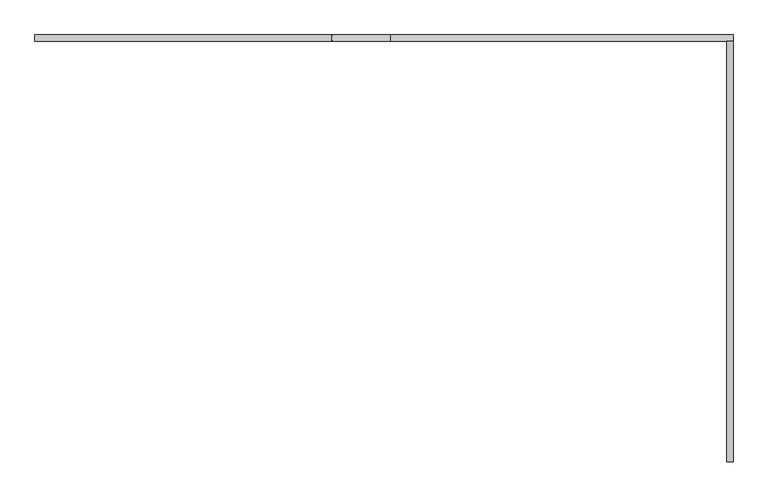
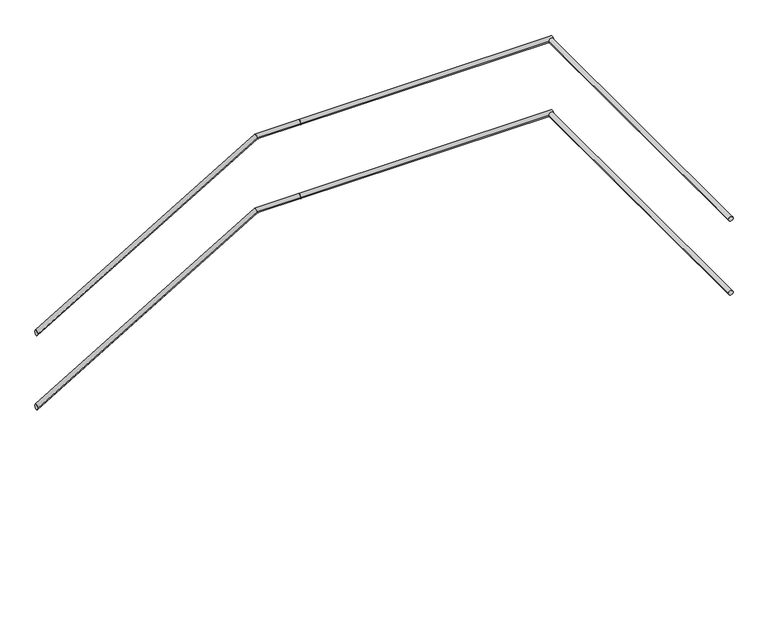
"""IFC4 building model written with IfcOpenShell, lengths in millimetres: railing geometry."""

import ifcopenshell
import ifcopenshell.guid

model = None  # the IFC model being written
_history = None  # IfcOwnerHistory: only IFC2X3 demands one
_inside = {}  # id of a spatial element -> (the spatial element, [elements in it])
_under = {}  # id of a project, library or spatial element -> (it, [spatial elements below it])
_declared = {}  # id of a project -> (the project, [libraries it declares])
_typed = {}  # id of a type object -> (the type object, [elements of that type])
_made_of = {}  # id of a material, layer set ... -> (it, [elements and type objects made of it])


def new_model(schema):
    """Start an empty IFC model of exactly this schema.

    Asked for "IFC4X3", IfcOpenShell would pick the latest addendum, in which some entities
    have other attributes; the version numbers below select the first issue.
    IFC2X3 requires an IfcOwnerHistory on every rooted entity: one is made here for all.
    """
    global model, _history
    if schema == "IFC4X3":
        model = ifcopenshell.file(schema_version=(4, 3, 0, 0))
    else:
        model = ifcopenshell.file(schema=schema)
    _inside.clear()
    _under.clear()
    _declared.clear()
    _typed.clear()
    _made_of.clear()
    _history = None
    if model.schema == "IFC2X3":
        org = make("IfcOrganization", Name="unknown")
        user = make(
            "IfcPersonAndOrganization",
            ThePerson=make("IfcPerson", FamilyName="unknown"),
            TheOrganization=org,
        )
        app = make(
            "IfcApplication",
            ApplicationDeveloper=org,
            Version="unknown",
            ApplicationFullName="unknown",
            ApplicationIdentifier="unknown",
        )
        _history = make(
            "IfcOwnerHistory",
            OwningUser=user,
            OwningApplication=app,
            ChangeAction="ADDED",
            CreationDate=0,
        )
    return model


def make(cls, **values):
    """One entity of the class cls with the attributes given. An attribute that is None is left unset."""
    return model.create_entity(
        cls, **{name: value for name, value in values.items() if value is not None}
    )


def rooted(cls, **values):
    """An entity with a GlobalId (a new one), such as an element, a storey or a relation."""
    return make(cls, GlobalId=ifcopenshell.guid.new(), OwnerHistory=_history, **values)


def si_unit(unit_type, name, prefix=None):
    """IfcSIUnit, for example si_unit("LENGTHUNIT", "METRE", prefix="MILLI")."""
    return make("IfcSIUnit", UnitType=unit_type, Prefix=prefix, Name=name)


def assignment(units):
    """IfcUnitAssignment: the units of a project."""
    return None if units is None else make("IfcUnitAssignment", Units=units)


def point(xyz):
    """IfcCartesianPoint."""
    return None if xyz is None else make("IfcCartesianPoint", Coordinates=xyz)


def direction(xyz):
    """IfcDirection."""
    return None if xyz is None else make("IfcDirection", DirectionRatios=xyz)


def frame(location, z_axis=None, x_axis=None):
    """IfcAxis2Placement3D, a coordinate frame: its origin and axes. An axis left out is left unset."""
    return make(
        "IfcAxis2Placement3D",
        Location=point(location),
        Axis=direction(z_axis),
        RefDirection=direction(x_axis),
    )


def origin():
    """The frame at (0, 0, 0) with its axes left unset."""
    return frame((0.0, 0.0, 0.0))


def place(relative_to, where):
    """IfcLocalPlacement: puts the frame where relative to a parent placement (None: the world)."""
    return make(
        "IfcLocalPlacement", PlacementRelTo=relative_to, RelativePlacement=where
    )


def context(
    kind, dimensions, precision=None, world=None, true_north=None, identifier=None
):
    """IfcGeometricRepresentationContext, for example the 3D "Model" context."""
    return make(
        "IfcGeometricRepresentationContext",
        ContextIdentifier=identifier,
        ContextType=kind,
        CoordinateSpaceDimension=dimensions,
        Precision=precision,
        WorldCoordinateSystem=world,
        TrueNorth=true_north,
    )


def project(units=None, contexts=None):
    """IfcProject with its units and contexts."""
    return rooted(
        "IfcProject",
        Name="project",
        RepresentationContexts=contexts,
        UnitsInContext=assignment(units),
    )


def spatial(cls, under=None, at=None, **own):
    """A site, building, storey or space (cls), placed at a placement, below another one or the project."""
    s = rooted(cls, ObjectPlacement=at, **own)
    if under is not None:
        _under.setdefault(under.id(), (under, []))[1].append(s)
    return s


def circle_curve(where, radius):
    """IfcCircle in the frame where."""
    return make("IfcCircle", Position=where, Radius=radius)


def ellipse_curve(where, semi_axis1, semi_axis2):
    """IfcEllipse in the frame where."""
    return make(
        "IfcEllipse", Position=where, SemiAxis1=semi_axis1, SemiAxis2=semi_axis2
    )


def shape(context_of_items, identifier, shape_type, items):
    """IfcShapeRepresentation: the items that make up one representation, for example the "Body"."""
    return make(
        "IfcShapeRepresentation",
        ContextOfItems=context_of_items,
        RepresentationIdentifier=identifier,
        RepresentationType=shape_type,
        Items=items,
    )


def source(mapping_origin, context_of_items, identifier, shape_type, items):
    """IfcRepresentationMap: a shape defined once, which mapped items show again and again."""
    return make(
        "IfcRepresentationMap",
        MappingOrigin=mapping_origin,
        MappedRepresentation=shape(context_of_items, identifier, shape_type, items),
    )


def transform(
    local_origin,
    x_axis=None,
    y_axis=None,
    z_axis=None,
    scale=None,
    scale2=None,
    scale3=None,
    uniform=True,
):
    """IfcCartesianTransformationOperator3D, or its non-uniform kind. x_axis, y_axis, z_axis: its Axis1, 2, 3."""
    if uniform:
        return make(
            "IfcCartesianTransformationOperator3D",
            Axis1=direction(x_axis),
            Axis2=direction(y_axis),
            LocalOrigin=point(local_origin),
            Scale=scale,
            Axis3=direction(z_axis),
        )
    return make(
        "IfcCartesianTransformationOperator3DnonUniform",
        Axis1=direction(x_axis),
        Axis2=direction(y_axis),
        LocalOrigin=point(local_origin),
        Scale=scale,
        Axis3=direction(z_axis),
        Scale2=scale2,
        Scale3=scale3,
    )


def mapped(mapping_source, mapping_target):
    """IfcMappedItem: shows the shape of a source again, moved by a transform."""
    return make(
        "IfcMappedItem", MappingSource=mapping_source, MappingTarget=mapping_target
    )


def made_of(thing, what):
    """Note that an element or type object is made of a material, layer set ...; save() writes the relation."""
    if what is not None:
        _made_of.setdefault(what.id(), (what, []))[1].append(thing)
    return thing


def element(
    cls,
    number,
    at=None,
    inside=None,
    cuts=None,
    type_object=None,
    material=None,
    context=None,
    identifier="Body",
    shape_type=None,
    held_by="IfcProductDefinitionShape",
    body=None,
    shapes=None,
    **own,
):
    """One element of the class cls, such as IfcWall. Its Tag is "e" and its number.

    at: its placement. inside: the storey or other place that contains it. cuts: it is an
    opening in that element (IfcRelVoidsElement). A single representation is given by context,
    identifier, shape_type and body (its items); several are given by shapes. held_by: the class
    of the entity that holds the representations. save() writes the other relations.
    """
    e = rooted(cls, Tag="e%d" % number, ObjectPlacement=at, **own)
    if body is not None:
        shapes = [shape(context, identifier, shape_type, body)]
    if shapes is not None:
        e.Representation = make(held_by, Representations=shapes)
    if inside is not None:
        _inside.setdefault(inside.id(), (inside, []))[1].append(e)
    if cuts is not None:
        rooted(
            "IfcRelVoidsElement", RelatingBuildingElement=cuts, RelatedOpeningElement=e
        )
    if type_object is not None:
        _typed.setdefault(type_object.id(), (type_object, []))[1].append(e)
    return made_of(e, material)


def aggregate(whole, parts):
    """IfcRelAggregates: a whole, such as a stair, and the parts it consists of."""
    return rooted("IfcRelAggregates", RelatingObject=whole, RelatedObjects=parts)


def save(model, path):
    """Write the relations noted so far, then the file.

    IfcRelAggregates (storeys below a building ...), IfcRelContainedInSpatialStructure (elements
    in a storey), IfcRelDefinesByType, IfcRelAssociatesMaterial and IfcRelDeclares: one each for
    every whole, place, type object, material and project.
    """
    for whole, parts in _under.values():
        aggregate(whole, parts)
    for where, things in _inside.values():
        rooted(
            "IfcRelContainedInSpatialStructure",
            RelatedElements=things,
            RelatingStructure=where,
        )
    for kind, things in _typed.values():
        rooted("IfcRelDefinesByType", RelatedObjects=things, RelatingType=kind)
    for what, things in _made_of.values():
        rooted("IfcRelAssociatesMaterial", RelatedObjects=things, RelatingMaterial=what)
    for by, libraries in _declared.values():
        rooted("IfcRelDeclares", RelatingContext=by, RelatedDefinitions=libraries)
    model.write(path)


def plane_surface(at):
    """IfcPlane: the flat surface through the origin of the frame at, square to its z axis."""
    return make("IfcPlane", Position=at)


def cylinder_surface(at, radius):
    """IfcCylindricalSurface: all points at the distance radius from the z axis of the frame at."""
    return make("IfcCylindricalSurface", Position=at, Radius=radius)


def advanced_brep(points, edges, surfaces, faces):
    """IfcAdvancedBrep: a solid bounded by faces that lie on surfaces and meet in shared edges.

    An edge is (start, end): straight between two places in points (the first is 0);
    or (start, end, curve); or (start, end, curve, False) where it runs against its curve.
    A face is (place in surfaces, loops), or (place, loops, False) where it looks against
    its surface's normal. A loop lists edges by number (the first is 1), with a minus sign
    where the edge is run from its end to its start. The first loop is the outer one.
    """
    corners = [point(p) for p in points]
    vertices = [make("IfcVertexPoint", VertexGeometry=c) for c in corners]
    made = []
    for start, end, *more in edges:
        made.append(
            make(
                "IfcEdgeCurve",
                EdgeStart=vertices[start],
                EdgeEnd=vertices[end],
                EdgeGeometry=more[0] if more else make("IfcPolyline", Points=[corners[start], corners[end]]),
                SameSense=more[1] if len(more) > 1 else True,
            )
        )
    hull = []
    for where, loops, *sense in faces:
        bounds = []
        for j, loop in enumerate(loops):
            ring = [make("IfcOrientedEdge", EdgeElement=made[abs(k) - 1], Orientation=k > 0) for k in loop]
            bounds.append(
                make(
                    "IfcFaceOuterBound" if j == 0 else "IfcFaceBound",
                    Bound=make("IfcEdgeLoop", EdgeList=ring),
                    Orientation=True,
                )
            )
        hull.append(make("IfcAdvancedFace", Bounds=bounds, FaceSurface=surfaces[where], SameSense=sense[0] if sense else True))
    return make("IfcAdvancedBrep", Outer=make("IfcClosedShell", CfsFaces=hull))


def railing_b1a865fd(model_context):
    return source(origin(), model_context, "Body", "AdvancedBrep", [
        advanced_brep(
        [(45466.7161135, 23749.5208589, 1734.9618634), (45496.7161135, 23749.5208589, 1734.9618634), (45466.7161135, 25734.1208589, 1734.9618634), (45496.7161135, 25734.1208589, 1734.9618634)],
        [
            (0, 1, circle_curve(frame((45481.7161135, 23749.5208589, 1734.9618634), z_axis=(0.0, -1.0, 0.0), x_axis=(1.0, 0.0, 0.0)), 15.0)),
            (1, 0, circle_curve(frame((45481.7161135, 23749.5208589, 1734.9618634), z_axis=(0.0, -1.0, 0.0), x_axis=(1.0, 0.0, 0.0)), 15.0)),
            (2, 3, circle_curve(frame((45481.7161135, 25734.1208589, 1734.9618634), z_axis=(0.0, 1.0, 0.0), x_axis=(1.0, 0.0, 0.0)), 15.0)),
            (3, 2, circle_curve(frame((45481.7161135, 25734.1208589, 1734.9618634), z_axis=(0.0, 1.0, 0.0), x_axis=(1.0, 0.0, 0.0)), 15.0)),
            (0, 2),
            (3, 1),
        ],
        [
            plane_surface(frame((45481.7161135, 23749.5208589, 1749.9618634), z_axis=(0.0, -1.0, 0.0), x_axis=(0.0, 0.0, 1.0))),
            plane_surface(frame((45481.7161135, 25734.1208589, 1749.9618634), z_axis=(0.0, 1.0, 0.0), x_axis=(0.0, 0.0, 1.0))),
            cylinder_surface(frame((45481.7161135, 23749.5208589, 1734.9618634), z_axis=(0.0, -1.0, 0.0), x_axis=(1.0, 0.0, 0.0)), 15.0),
        ],
        [
            (0, [[1, 2]]),
            (1, [[3, 4]]),
            (2, [[-1, 5, -4, 6]]),
            (2, [[-2, -6, -3, -5]]),
        ],
    ),
        advanced_brep(
        [(45496.7161135, 25734.1208589, 1734.9618634), (45496.7161135, 25764.1208589, 1734.9618634), (43882.1161135, 25734.1208589, 1734.9618634), (43882.1161135, 25764.1208589, 1734.9618634)],
        [
            (0, 1, circle_curve(frame((45496.7161135, 25749.1208589, 1734.9618634), z_axis=(1.0, 0.0, 0.0), x_axis=(0.0, 1.0, 0.0)), 15.0)),
            (1, 0, circle_curve(frame((45496.7161135, 25749.1208589, 1734.9618634), z_axis=(1.0, 0.0, 0.0), x_axis=(0.0, 1.0, 0.0)), 15.0)),
            (2, 3, circle_curve(frame((43882.1161135, 25749.1208589, 1734.9618634), z_axis=(-1.0, 0.0, 0.0), x_axis=(0.0, 1.0, 0.0)), 15.0)),
            (3, 2, circle_curve(frame((43882.1161135, 25749.1208589, 1734.9618634), z_axis=(-1.0, 0.0, 0.0), x_axis=(0.0, 1.0, 0.0)), 15.0)),
            (0, 2),
            (3, 1),
        ],
        [
            plane_surface(frame((45496.7161135, 25749.1208589, 1749.9618634), z_axis=(1.0, 0.0, 0.0), x_axis=(0.0, -1.0, 0.0))),
            plane_surface(frame((43882.1161135, 25749.1208589, 1749.9618634), z_axis=(-1.0, 0.0, 0.0), x_axis=(0.0, -1.0, 0.0))),
            cylinder_surface(frame((45496.7161135, 25749.1208589, 1734.9618634), z_axis=(1.0, 0.0, 0.0), x_axis=(0.0, 1.0, 0.0)), 15.0),
        ],
        [
            (0, [[1, 2]]),
            (1, [[3, 4]]),
            (2, [[-1, 5, -4, 6]]),
            (2, [[-2, -6, -3, -5]]),
        ],
    ),
        advanced_brep(
        [(43882.1161135, 25734.1208589, 1734.9618634), (43882.1161135, 25764.1208589, 1734.9618634), (43606.242552, 25734.1208589, 1734.9618634), (43606.242552, 25764.1208589, 1734.9618634), (42202.1161135, 25734.1208589, 899.1723166), (42202.1161135, 25764.1208589, 899.1723166)],
        [
            (0, 1, circle_curve(frame((43882.1161135, 25749.1208589, 1734.9618634), z_axis=(1.0, 0.0, 0.0), x_axis=(0.0, 1.0, 0.0)), 15.0)),
            (1, 0, circle_curve(frame((43882.1161135, 25749.1208589, 1734.9618634), z_axis=(1.0, 0.0, 0.0), x_axis=(0.0, 1.0, 0.0)), 15.0)),
            (0, 2),
            (2, 3, ellipse_curve(frame((43606.242552, 25749.1208589, 1734.9618634), z_axis=(0.9641817474962143, 0.0, 0.2652424509673111), x_axis=(0.265242450967311, 0.0, -0.9641817474962144)), 15.5572329, 15.0)),
            (3, 1),
            (3, 2, ellipse_curve(frame((43606.242552, 25749.1208589, 1734.9618634), z_axis=(0.9641817474962143, 0.0, 0.2652424509673111), x_axis=(0.265242450967311, 0.0, -0.9641817474962144)), 15.5572329, 15.0)),
            (4, 5, ellipse_curve(frame((42202.1161135, 25749.1208589, 899.1723166), z_axis=(-1.0, 0.0, 0.0), x_axis=(0.0, 0.0, 1.0)), 17.4562134, 15.0)),
            (5, 4, ellipse_curve(frame((42202.1161135, 25749.1208589, 899.1723166), z_axis=(-1.0, 0.0, 0.0), x_axis=(0.0, 0.0, 1.0)), 17.4562134, 15.0)),
            (2, 4),
            (5, 3),
        ],
        [
            plane_surface(frame((43882.1161135, 25749.1208589, 1749.9618634), z_axis=(1.0, 0.0, 0.0), x_axis=(0.0, -1.0, 0.0))),
            cylinder_surface(frame((43882.1161135, 25749.1208589, 1734.9618634), z_axis=(1.0, 0.0, 0.0), x_axis=(0.0, 1.0, 0.0)), 15.0),
            plane_surface(frame((42202.1161135, 25749.1208589, 916.62853), z_axis=(-1.0, 0.0, 0.0), x_axis=(0.0, -1.0, 0.0))),
            cylinder_surface(frame((43609.7883714, 25749.1208589, 1737.0724701), z_axis=(0.8592928844097072, 0.0, 0.5114838597676818), x_axis=(0.0, 1.0, 0.0)), 15.0),
        ],
        [
            (0, [[1, 2]]),
            (1, [[-1, 3, 4, 5]]),
            (1, [[-2, -5, 6, -3]]),
            (2, [[7, 8]]),
            (3, [[-4, 9, -8, 10]]),
            (3, [[-6, -10, -7, -9]]),
        ],
    ),
        advanced_brep(
        [(45466.7161135, 23749.5208589, 2234.9618634), (45496.7161135, 23749.5208589, 2234.9618634), (45466.7161135, 25734.1208589, 2234.9618634), (45496.7161135, 25734.1208589, 2234.9618634)],
        [
            (0, 1, circle_curve(frame((45481.7161135, 23749.5208589, 2234.9618634), z_axis=(0.0, -1.0, 0.0), x_axis=(1.0, 0.0, 0.0)), 15.0)),
            (1, 0, circle_curve(frame((45481.7161135, 23749.5208589, 2234.9618634), z_axis=(0.0, -1.0, 0.0), x_axis=(1.0, 0.0, 0.0)), 15.0)),
            (2, 3, circle_curve(frame((45481.7161135, 25734.1208589, 2234.9618634), z_axis=(0.0, 1.0, 0.0), x_axis=(1.0, 0.0, 0.0)), 15.0)),
            (3, 2, circle_curve(frame((45481.7161135, 25734.1208589, 2234.9618634), z_axis=(0.0, 1.0, 0.0), x_axis=(1.0, 0.0, 0.0)), 15.0)),
            (0, 2),
            (3, 1),
        ],
        [
            plane_surface(frame((45481.7161135, 23749.5208589, 2249.9618634), z_axis=(0.0, -1.0, 0.0), x_axis=(0.0, 0.0, 1.0))),
            plane_surface(frame((45481.7161135, 25734.1208589, 2249.9618634), z_axis=(0.0, 1.0, 0.0), x_axis=(0.0, 0.0, 1.0))),
            cylinder_surface(frame((45481.7161135, 23749.5208589, 2234.9618634), z_axis=(0.0, -1.0, 0.0), x_axis=(1.0, 0.0, 0.0)), 15.0),
        ],
        [
            (0, [[1, 2]]),
            (1, [[3, 4]]),
            (2, [[-1, 5, -4, 6]]),
            (2, [[-2, -6, -3, -5]]),
        ],
    ),
        advanced_brep(
        [(45496.7161135, 25734.1208589, 2234.9618634), (45496.7161135, 25764.1208589, 2234.9618634), (43882.1161135, 25734.1208589, 2234.9618634), (43882.1161135, 25764.1208589, 2234.9618634)],
        [
            (0, 1, circle_curve(frame((45496.7161135, 25749.1208589, 2234.9618634), z_axis=(1.0, 0.0, 0.0), x_axis=(0.0, 1.0, 0.0)), 15.0)),
            (1, 0, circle_curve(frame((45496.7161135, 25749.1208589, 2234.9618634), z_axis=(1.0, 0.0, 0.0), x_axis=(0.0, 1.0, 0.0)), 15.0)),
            (2, 3, circle_curve(frame((43882.1161135, 25749.1208589, 2234.9618634), z_axis=(-1.0, 0.0, 0.0), x_axis=(0.0, 1.0, 0.0)), 15.0)),
            (3, 2, circle_curve(frame((43882.1161135, 25749.1208589, 2234.9618634), z_axis=(-1.0, 0.0, 0.0), x_axis=(0.0, 1.0, 0.0)), 15.0)),
            (0, 2),
            (3, 1),
        ],
        [
            plane_surface(frame((45496.7161135, 25749.1208589, 2249.9618634), z_axis=(1.0, 0.0, 0.0), x_axis=(0.0, -1.0, 0.0))),
            plane_surface(frame((43882.1161135, 25749.1208589, 2249.9618634), z_axis=(-1.0, 0.0, 0.0), x_axis=(0.0, -1.0, 0.0))),
            cylinder_surface(frame((45496.7161135, 25749.1208589, 2234.9618634), z_axis=(1.0, 0.0, 0.0), x_axis=(0.0, 1.0, 0.0)), 15.0),
        ],
        [
            (0, [[1, 2]]),
            (1, [[3, 4]]),
            (2, [[-1, 5, -4, 6]]),
            (2, [[-2, -6, -3, -5]]),
        ],
    ),
        advanced_brep(
        [(43882.1161135, 25734.1208589, 2234.9618634), (43882.1161135, 25764.1208589, 2234.9618634), (43606.242552, 25734.1208589, 2234.9618634), (43606.242552, 25764.1208589, 2234.9618634), (42202.1161135, 25734.1208589, 1399.1723166), (42202.1161135, 25764.1208589, 1399.1723166)],
        [
            (0, 1, circle_curve(frame((43882.1161135, 25749.1208589, 2234.9618634), z_axis=(1.0, 0.0, 0.0), x_axis=(0.0, 1.0, 0.0)), 15.0)),
            (1, 0, circle_curve(frame((43882.1161135, 25749.1208589, 2234.9618634), z_axis=(1.0, 0.0, 0.0), x_axis=(0.0, 1.0, 0.0)), 15.0)),
            (0, 2),
            (2, 3, ellipse_curve(frame((43606.242552, 25749.1208589, 2234.9618634), z_axis=(0.9641817474962143, 0.0, 0.2652424509673111), x_axis=(0.265242450967311, 0.0, -0.9641817474962144)), 15.5572329, 15.0)),
            (3, 1),
            (3, 2, ellipse_curve(frame((43606.242552, 25749.1208589, 2234.9618634), z_axis=(0.9641817474962143, 0.0, 0.2652424509673111), x_axis=(0.265242450967311, 0.0, -0.9641817474962144)), 15.5572329, 15.0)),
            (4, 5, ellipse_curve(frame((42202.1161135, 25749.1208589, 1399.1723166), z_axis=(-1.0, 0.0, 0.0), x_axis=(0.0, 0.0, 1.0)), 17.4562134, 15.0)),
            (5, 4, ellipse_curve(frame((42202.1161135, 25749.1208589, 1399.1723166), z_axis=(-1.0, 0.0, 0.0), x_axis=(0.0, 0.0, 1.0)), 17.4562134, 15.0)),
            (2, 4),
            (5, 3),
        ],
        [
            plane_surface(frame((43882.1161135, 25749.1208589, 2249.9618634), z_axis=(1.0, 0.0, 0.0), x_axis=(0.0, -1.0, 0.0))),
            cylinder_surface(frame((43882.1161135, 25749.1208589, 2234.9618634), z_axis=(1.0, 0.0, 0.0), x_axis=(0.0, 1.0, 0.0)), 15.0),
            plane_surface(frame((42202.1161135, 25749.1208589, 1416.62853), z_axis=(-1.0, 0.0, 0.0), x_axis=(0.0, -1.0, 0.0))),
            cylinder_surface(frame((43609.7883714, 25749.1208589, 2237.0724701), z_axis=(0.8592928844097072, 0.0, 0.5114838597676818), x_axis=(0.0, 1.0, 0.0)), 15.0),
        ],
        [
            (0, [[1, 2]]),
            (1, [[-1, 3, 4, 5]]),
            (1, [[-2, -5, 6, -3]]),
            (2, [[7, 8]]),
            (3, [[-4, 9, -8, 10]]),
            (3, [[-6, -10, -7, -9]]),
        ],
    ),
    ])


if __name__ == "__main__":
    model = new_model("IFC4")
    model_context = context("Model", 3, world=origin())
    ifc_project = project(units=[si_unit("LENGTHUNIT", "METRE", prefix="MILLI")], contexts=[model_context])
    site = spatial("IfcSite", under=ifc_project)
    building = spatial("IfcBuilding", under=site)
    placement = place(None, origin())
    railing_shape = railing_b1a865fd(model_context)
    element("IfcRailing", 1, at=placement, inside=building, context=model_context, shape_type="MappedRepresentation", body=[
        mapped(railing_shape, transform((0.0, 0.0, 0.0), x_axis=(1.0, 0.0, 0.0), y_axis=(0.0, 1.0, 0.0), z_axis=(0.0, 0.0, 1.0))),
    ])
    save(model, "model.ifc")
